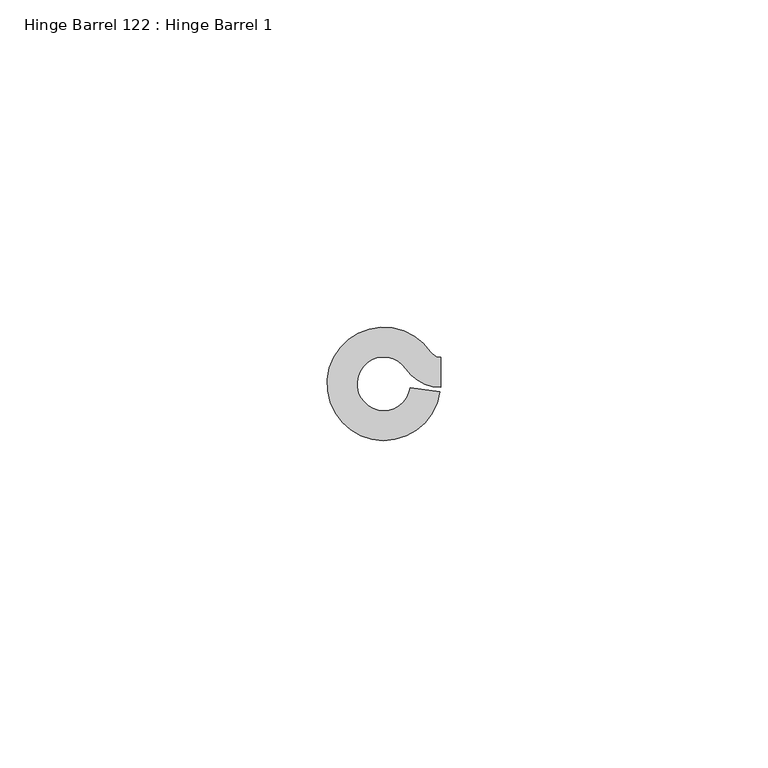
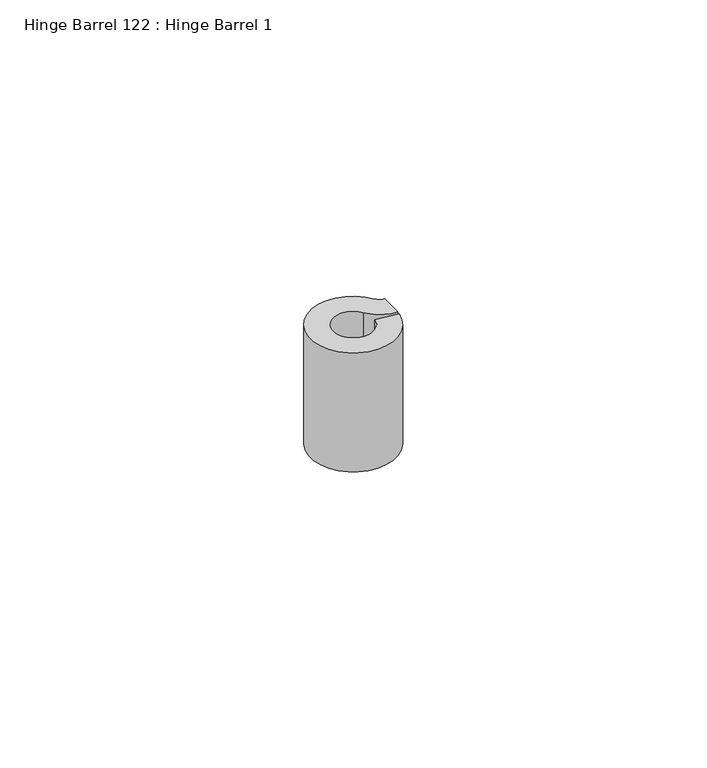
"""IFC4 building model written with IfcOpenShell, lengths in millimetres: proxy geometry, Hinge Barrel 122 : Hinge Barrel 1."""

from ifc_helpers import new_model, si_unit, point, frame, frame_2d, origin, place, context, project, spatial, polyline, circle_curve, trimmed, segment, composite_curve, outline, extrude, source, transform, mapped, element, save


def hinge_barrel_122_hinge_barrel_1_a09c7832(model_context):
    return source(origin(), model_context, "Body", "SweptSolid", [
        extrude(outline(composite_curve([segment(trimmed(circle_curve(frame_2d((587319.1320739, -534100.7049841)), 4.0894), [point((587322.5194669, -534098.4139665))], [point((587323.1821338, -534101.2708529))], True, "CARTESIAN"), True, "CONTINUOUS"), segment(polyline([(587323.1821338, -534101.2708529), (587327.7022899, -534101.9024028)]), True, "CONTINUOUS"), segment(trimmed(circle_curve(frame_2d((587319.1320739, -534100.7049841)), 8.6534625), [point((587327.7022899, -534101.9024028))], [point((587326.3000393, -534095.8570273))], False, "CARTESIAN"), True, "CONTINUOUS"), segment(trimmed(circle_curve(frame_2d((587327.8245257, -534094.8259615)), 1.8404226), [point((587326.3000393, -534095.8570273))], [point((587327.8245257, -534096.6663841))], True, "CARTESIAN"), True, "CONTINUOUS"), segment(polyline([(587327.8245257, -534096.6663841), (587327.8245257, -534101.2304466)]), True, "CONTINUOUS"), segment(trimmed(circle_curve(frame_2d((587327.8245257, -534094.8259615)), 6.4044851), [point((587327.8245257, -534101.2304466))], [point((587322.5194669, -534098.4139665))], False, "CARTESIAN"), True, "CONTINUOUS")], self_intersect=False)), frame((0.0, 0.0, 1149.35), z_axis=(0.0, 0.0, 1.0), x_axis=(1.0, 0.0, 0.0)), (0.0, 0.0, 1.0), 25.4),
    ])


if __name__ == "__main__":
    model = new_model("IFC4")
    model_context = context("Model", 3, world=origin())
    ifc_project = project(units=[si_unit("LENGTHUNIT", "METRE", prefix="MILLI")], contexts=[model_context])
    site = spatial("IfcSite", under=ifc_project)
    building = spatial("IfcBuilding", under=site)
    placement = place(None, origin())
    hinge_barrel_122_hinge_barrel_1_shape = hinge_barrel_122_hinge_barrel_1_a09c7832(model_context)
    element("IfcBuildingElementProxy", 1, Name="Hinge Barrel 122 : Hinge Barrel 1", ObjectType="Hinge Barrel 122 : Hinge Barrel 1", at=placement, inside=building, context=model_context, shape_type="MappedRepresentation", body=[
        mapped(hinge_barrel_122_hinge_barrel_1_shape, transform((0.0, 0.0, 0.0), x_axis=(1.0, 0.0, 0.0), y_axis=(0.0, 1.0, 0.0), z_axis=(0.0, 0.0, 1.0))),
    ])
    save(model, "model.ifc")

# Revit data of these elements
# Element 1 (IfcBuildingElementProxy, "Hinge Barrel 122 : Hinge Barrel 1")
#   Materials on its faces: "6\"X6\" WELD-ON STL BUTT HINGE"
# Materials
#   "6\"X6\" WELD-ON STL BUTT HINGE": class "Metal", colour RGB 189 187 185, transparency 0, Description = "Carbon steel", Cost = 0
